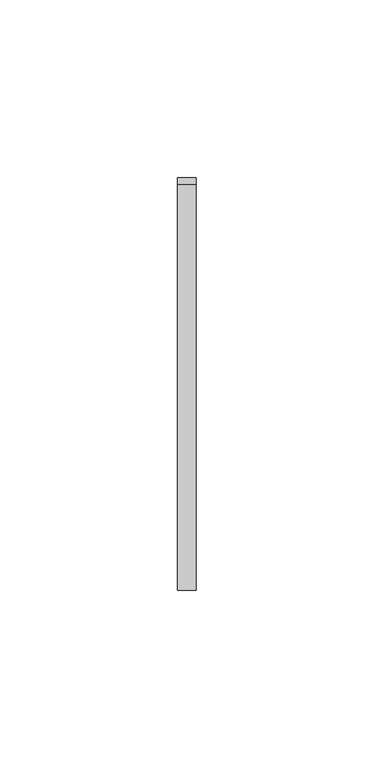
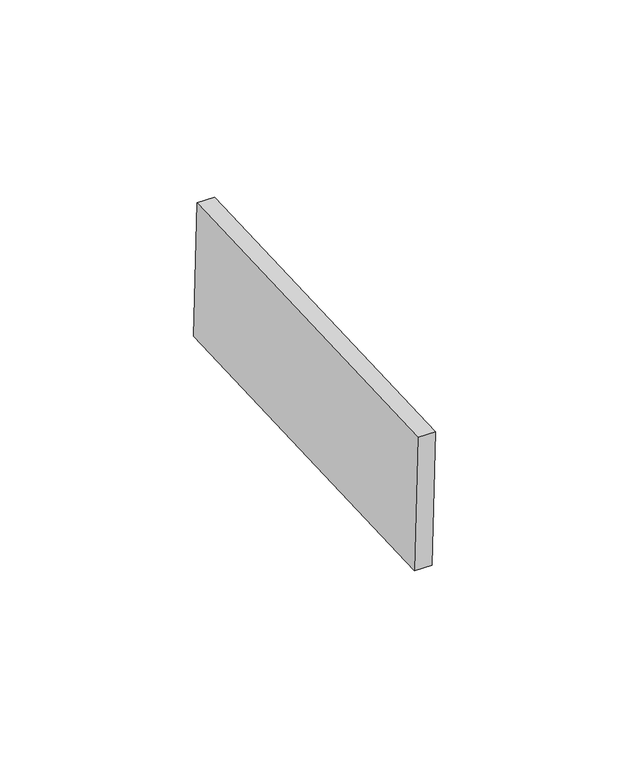
"""IFC4 building model written with IfcOpenShell, lengths in millimetres: proxy geometry, Inner panel:Inner panel:1:Inner panel:1 : Inner panel:Inner panel:300324:2:Inner panel:1:Inner panel:1 : Inner panel:Inner panel:300324:2 : Inner panel:Inner panel:1:Inner panel:1 : Inner panel:Inner panel:300324:300043:44 : Inner panel:Inner panel:1:Inner panel:1 : Inner panel:Inner panel:300324:2:Inner panel:1:Inner panel:1 : Inner panel:Inner panel:300324:2 : Inner panel:Inner panel:1:Inner panel:1 : Inner panel:Inner panel:300324:300043:308120."""

import ifcopenshell
import ifcopenshell.guid

model = None  # the IFC model being written
_history = None  # IfcOwnerHistory: only IFC2X3 demands one
_inside = {}  # id of a spatial element -> (the spatial element, [elements in it])
_under = {}  # id of a project, library or spatial element -> (it, [spatial elements below it])
_declared = {}  # id of a project -> (the project, [libraries it declares])
_typed = {}  # id of a type object -> (the type object, [elements of that type])
_made_of = {}  # id of a material, layer set ... -> (it, [elements and type objects made of it])


def new_model(schema):
    """Start an empty IFC model of exactly this schema.

    Asked for "IFC4X3", IfcOpenShell would pick the latest addendum, in which some entities
    have other attributes; the version numbers below select the first issue.
    IFC2X3 requires an IfcOwnerHistory on every rooted entity: one is made here for all.
    """
    global model, _history
    if schema == "IFC4X3":
        model = ifcopenshell.file(schema_version=(4, 3, 0, 0))
    else:
        model = ifcopenshell.file(schema=schema)
    _inside.clear()
    _under.clear()
    _declared.clear()
    _typed.clear()
    _made_of.clear()
    _history = None
    if model.schema == "IFC2X3":
        org = make("IfcOrganization", Name="unknown")
        user = make(
            "IfcPersonAndOrganization",
            ThePerson=make("IfcPerson", FamilyName="unknown"),
            TheOrganization=org,
        )
        app = make(
            "IfcApplication",
            ApplicationDeveloper=org,
            Version="unknown",
            ApplicationFullName="unknown",
            ApplicationIdentifier="unknown",
        )
        _history = make(
            "IfcOwnerHistory",
            OwningUser=user,
            OwningApplication=app,
            ChangeAction="ADDED",
            CreationDate=0,
        )
    return model


def make(cls, **values):
    """One entity of the class cls with the attributes given. An attribute that is None is left unset."""
    return model.create_entity(
        cls, **{name: value for name, value in values.items() if value is not None}
    )


def rooted(cls, **values):
    """An entity with a GlobalId (a new one), such as an element, a storey or a relation."""
    return make(cls, GlobalId=ifcopenshell.guid.new(), OwnerHistory=_history, **values)


def si_unit(unit_type, name, prefix=None):
    """IfcSIUnit, for example si_unit("LENGTHUNIT", "METRE", prefix="MILLI")."""
    return make("IfcSIUnit", UnitType=unit_type, Prefix=prefix, Name=name)


def assignment(units):
    """IfcUnitAssignment: the units of a project."""
    return None if units is None else make("IfcUnitAssignment", Units=units)


def point(xyz):
    """IfcCartesianPoint."""
    return None if xyz is None else make("IfcCartesianPoint", Coordinates=xyz)


def direction(xyz):
    """IfcDirection."""
    return None if xyz is None else make("IfcDirection", DirectionRatios=xyz)


def frame(location, z_axis=None, x_axis=None):
    """IfcAxis2Placement3D, a coordinate frame: its origin and axes. An axis left out is left unset."""
    return make(
        "IfcAxis2Placement3D",
        Location=point(location),
        Axis=direction(z_axis),
        RefDirection=direction(x_axis),
    )


def origin():
    """The frame at (0, 0, 0) with its axes left unset."""
    return frame((0.0, 0.0, 0.0))


def place(relative_to, where):
    """IfcLocalPlacement: puts the frame where relative to a parent placement (None: the world)."""
    return make(
        "IfcLocalPlacement", PlacementRelTo=relative_to, RelativePlacement=where
    )


def context(
    kind, dimensions, precision=None, world=None, true_north=None, identifier=None
):
    """IfcGeometricRepresentationContext, for example the 3D "Model" context."""
    return make(
        "IfcGeometricRepresentationContext",
        ContextIdentifier=identifier,
        ContextType=kind,
        CoordinateSpaceDimension=dimensions,
        Precision=precision,
        WorldCoordinateSystem=world,
        TrueNorth=true_north,
    )


def project(units=None, contexts=None):
    """IfcProject with its units and contexts."""
    return rooted(
        "IfcProject",
        Name="project",
        RepresentationContexts=contexts,
        UnitsInContext=assignment(units),
    )


def spatial(cls, under=None, at=None, **own):
    """A site, building, storey or space (cls), placed at a placement, below another one or the project."""
    s = rooted(cls, ObjectPlacement=at, **own)
    if under is not None:
        _under.setdefault(under.id(), (under, []))[1].append(s)
    return s


def polyline(points):
    """IfcPolyline through the points."""
    return make("IfcPolyline", Points=[point(p) for p in points])


def outline(outer, holes=None, kind="AREA"):
    """IfcArbitraryClosedProfileDef: a profile drawn as a closed curve; with holes, ...WithVoids."""
    if holes is None:
        return make("IfcArbitraryClosedProfileDef", ProfileType=kind, OuterCurve=outer)
    return make(
        "IfcArbitraryProfileDefWithVoids",
        ProfileType=kind,
        OuterCurve=outer,
        InnerCurves=holes,
    )


def extrude(swept, where, along, depth):
    """IfcExtrudedAreaSolid: the profile swept, set in the frame where, extruded along a direction by depth."""
    return make(
        "IfcExtrudedAreaSolid",
        SweptArea=swept,
        Position=where,
        ExtrudedDirection=direction(along),
        Depth=depth,
    )


def shape(context_of_items, identifier, shape_type, items):
    """IfcShapeRepresentation: the items that make up one representation, for example the "Body"."""
    return make(
        "IfcShapeRepresentation",
        ContextOfItems=context_of_items,
        RepresentationIdentifier=identifier,
        RepresentationType=shape_type,
        Items=items,
    )


def source(mapping_origin, context_of_items, identifier, shape_type, items):
    """IfcRepresentationMap: a shape defined once, which mapped items show again and again."""
    return make(
        "IfcRepresentationMap",
        MappingOrigin=mapping_origin,
        MappedRepresentation=shape(context_of_items, identifier, shape_type, items),
    )


def transform(
    local_origin,
    x_axis=None,
    y_axis=None,
    z_axis=None,
    scale=None,
    scale2=None,
    scale3=None,
    uniform=True,
):
    """IfcCartesianTransformationOperator3D, or its non-uniform kind. x_axis, y_axis, z_axis: its Axis1, 2, 3."""
    if uniform:
        return make(
            "IfcCartesianTransformationOperator3D",
            Axis1=direction(x_axis),
            Axis2=direction(y_axis),
            LocalOrigin=point(local_origin),
            Scale=scale,
            Axis3=direction(z_axis),
        )
    return make(
        "IfcCartesianTransformationOperator3DnonUniform",
        Axis1=direction(x_axis),
        Axis2=direction(y_axis),
        LocalOrigin=point(local_origin),
        Scale=scale,
        Axis3=direction(z_axis),
        Scale2=scale2,
        Scale3=scale3,
    )


def mapped(mapping_source, mapping_target):
    """IfcMappedItem: shows the shape of a source again, moved by a transform."""
    return make(
        "IfcMappedItem", MappingSource=mapping_source, MappingTarget=mapping_target
    )


def made_of(thing, what):
    """Note that an element or type object is made of a material, layer set ...; save() writes the relation."""
    if what is not None:
        _made_of.setdefault(what.id(), (what, []))[1].append(thing)
    return thing


def element(
    cls,
    number,
    at=None,
    inside=None,
    cuts=None,
    type_object=None,
    material=None,
    context=None,
    identifier="Body",
    shape_type=None,
    held_by="IfcProductDefinitionShape",
    body=None,
    shapes=None,
    **own,
):
    """One element of the class cls, such as IfcWall. Its Tag is "e" and its number.

    at: its placement. inside: the storey or other place that contains it. cuts: it is an
    opening in that element (IfcRelVoidsElement). A single representation is given by context,
    identifier, shape_type and body (its items); several are given by shapes. held_by: the class
    of the entity that holds the representations. save() writes the other relations.
    """
    e = rooted(cls, Tag="e%d" % number, ObjectPlacement=at, **own)
    if body is not None:
        shapes = [shape(context, identifier, shape_type, body)]
    if shapes is not None:
        e.Representation = make(held_by, Representations=shapes)
    if inside is not None:
        _inside.setdefault(inside.id(), (inside, []))[1].append(e)
    if cuts is not None:
        rooted(
            "IfcRelVoidsElement", RelatingBuildingElement=cuts, RelatedOpeningElement=e
        )
    if type_object is not None:
        _typed.setdefault(type_object.id(), (type_object, []))[1].append(e)
    return made_of(e, material)


def aggregate(whole, parts):
    """IfcRelAggregates: a whole, such as a stair, and the parts it consists of."""
    return rooted("IfcRelAggregates", RelatingObject=whole, RelatedObjects=parts)


def save(model, path):
    """Write the relations noted so far, then the file.

    IfcRelAggregates (storeys below a building ...), IfcRelContainedInSpatialStructure (elements
    in a storey), IfcRelDefinesByType, IfcRelAssociatesMaterial and IfcRelDeclares: one each for
    every whole, place, type object, material and project.
    """
    for whole, parts in _under.values():
        aggregate(whole, parts)
    for where, things in _inside.values():
        rooted(
            "IfcRelContainedInSpatialStructure",
            RelatedElements=things,
            RelatingStructure=where,
        )
    for kind, things in _typed.values():
        rooted("IfcRelDefinesByType", RelatedObjects=things, RelatingType=kind)
    for what, things in _made_of.values():
        rooted("IfcRelAssociatesMaterial", RelatedObjects=things, RelatingMaterial=what)
    for by, libraries in _declared.values():
        rooted("IfcRelDeclares", RelatingContext=by, RelatedDefinitions=libraries)
    model.write(path)


def generic_models_b0fa762c(model_context):
    return source(origin(), model_context, "Body", "SweptSolid", [
        extrude(outline(polyline([(0.0, -114.3), (0.0, 0.0), (5.2138089, 0.0), (5.2138089, -114.3), (0.0, -114.3)])), frame((593530.195117, -577458.3096573, 4016.6427799), z_axis=(0.0, -0.04163054471216399, 0.9991330730923527), x_axis=(-1.0, 0.0, 0.0)), (0.0, 0.0, 1.0), 43.2233908),
    ])


if __name__ == "__main__":
    model = new_model("IFC4")
    model_context = context("Model", 3, world=origin())
    ifc_project = project(units=[si_unit("LENGTHUNIT", "METRE", prefix="MILLI")], contexts=[model_context])
    site = spatial("IfcSite", under=ifc_project)
    building = spatial("IfcBuilding", under=site)
    placement = place(None, origin())
    generic_models_shape = generic_models_b0fa762c(model_context)
    element("IfcBuildingElementProxy", 1, Name="Inner panel:Inner panel:1:Inner panel:1 : Inner panel:Inner panel:300324:2:Inner panel:1:Inner panel:1 : Inner panel:Inner panel:300324:2 : Inner panel:Inner panel:1:Inner panel:1 : Inner panel:Inner panel:300324:300043:44 : Inner panel:Inner panel:1:Inner panel:1 : Inner panel:Inner panel:300324:2:Inner panel:1:Inner panel:1 : Inner panel:Inner panel:300324:2 : Inner panel:Inner panel:1:Inner panel:1 : Inner panel:Inner panel:300324:300043:308120", ObjectType="Inner panel:Inner panel:1:Inner panel:1 : Inner panel:Inner panel:300324:2:Inner panel:1:Inner panel:1 : Inner panel:Inner panel:300324:2 : Inner panel:Inner panel:1:Inner panel:1 : Inner panel:Inner panel:300324:300043:44 : Inner panel:Inner panel:1:Inner panel:1 : Inner panel:Inner panel:300324:2:Inner panel:1:Inner panel:1 : Inner panel:Inner panel:300324:2 : Inner panel:Inner panel:1:Inner panel:1 : Inner panel:Inner panel:300324:300043:308120", at=placement, inside=building, context=model_context, shape_type="MappedRepresentation", body=[
        mapped(generic_models_shape, transform((0.0, 0.0, 0.0), x_axis=(1.0, 0.0, 0.0), y_axis=(0.0, 1.0, 0.0), z_axis=(0.0, 0.0, 1.0))),
    ])
    save(model, "model.ifc")

# Revit data of these elements
# Type "Inner panel:Inner panel:1:Inner panel:1 : Inner panel:Inner panel:300324:2:Inner panel:1:Inner panel:1 : Inner panel:Inner panel:300324:2 : Inner panel:Inner panel:1:Inner panel:1 : Inner panel:Inner panel:300324:300043:44 : Inner panel:Inner panel:1:Inner panel:1 : Inner panel:Inner panel:300324:2:Inner panel:1:Inner panel:1 : Inner panel:Inner panel:300324:2 : Inner panel:Inner panel:1:Inner panel:1 : Inner panel:Inner panel:300324:300043:308120"
#   NameOverride = "Inner panel:Inner panel:1:Inner panel:1 : Inner panel:Inner panel:300324:2:Inner panel:1:Inner panel:1 : Inner panel:Inner panel:300324:2 : Inner panel:Inner panel:1:Inner panel:1 : Inner panel:Inner panel:300324:300043:308120"
#   ObjectTypeOverride = "Inner panel:1:Inner panel:1 : Inner panel:Inner panel:300324:2 : Inner panel:Inner panel:1:Inner panel:1 : Inner panel:Inner panel:300324:300043"
#   Reference = "Inner panel"
#   Tag = "308120"
# Element 1 (IfcBuildingElementProxy, "Inner panel:Inner panel:1:Inner panel:1 : Inner panel:Inner panel:300324:2:Inner panel:1:Inner panel:1 : Inner panel:Inner panel:300324:2 : Inner panel:Inner panel:1:Inner panel:1 : Inner panel:Inner panel:300324:300043:44 : Inner panel:Inner panel:1:Inner panel:1 : Inner panel:Inner panel:300324:2:Inner panel:1:Inner panel:1 : Inner panel:Inner panel:300324:2 : Inner panel:Inner panel:1:Inner panel:1 : Inner panel:Inner panel:300324:300043:308120")
#   Materials on its faces: "SLIDING CLIP"
# Materials
#   "SLIDING CLIP": class "Generic", colour RGB 120 120 120, transparency 0, Cost = 0
